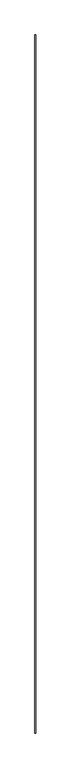
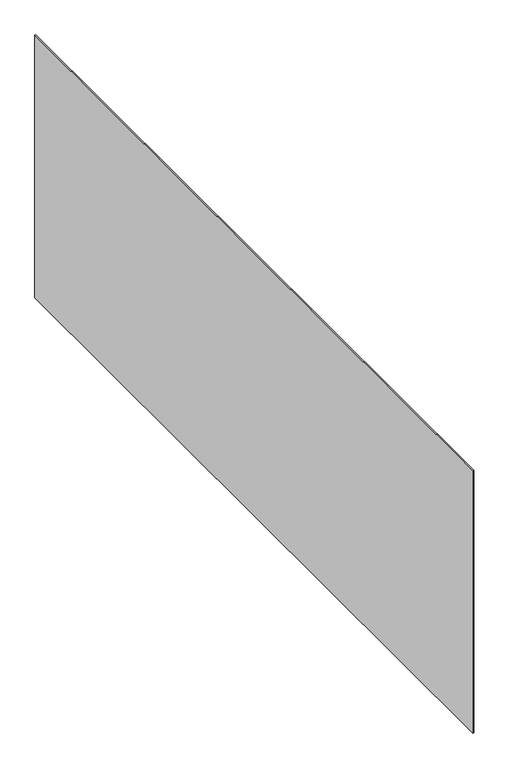
"""IFC4 building model written with IfcOpenShell, lengths in millimetres: proxy geometry, Panel:Panel:300402:Panel:300402 : Panel:Panel:300402:300124:Panel:300402:Panel:300402 : Panel:Panel:300402:300124 : Panel:Panel:300402:Panel:300402 : Panel:Panel:300402:300124:15 : Panel:Panel:300402:Panel:300402 : Panel:Panel:300402:300124:Panel:300402:Panel:300402 : Panel:Panel:300402:300124 : Panel:Panel:300402:Panel:300402 : Panel:Panel:300402:300124:300083."""

from ifc_helpers import new_model, si_unit, frame, origin, place, context, project, spatial, polyline, outline, extrude, source, transform, mapped, element, save


def generic_models_8c9edc3c(model_context):
    return source(origin(), model_context, "Body", "SweptSolid", [
        extrude(outline(polyline([(560264.0617239, -572944.1405465), (560264.0617239, -578718.1163841), (560256.1242239, -578718.1163841), (560256.1242239, -572944.1405465), (560264.0617239, -572944.1405465)])), frame((0.0, 0.0, 4023.758115), z_axis=(0.0, 0.0, 1.0), x_axis=(1.0, 0.0, 0.0)), (0.0, 0.0, 1.0), 2110.341885),
    ])


if __name__ == "__main__":
    model = new_model("IFC4")
    model_context = context("Model", 3, world=origin())
    ifc_project = project(units=[si_unit("LENGTHUNIT", "METRE", prefix="MILLI")], contexts=[model_context])
    site = spatial("IfcSite", under=ifc_project)
    building = spatial("IfcBuilding", under=site)
    placement = place(None, origin())
    generic_models_shape = generic_models_8c9edc3c(model_context)
    element("IfcBuildingElementProxy", 1, Name="Panel:Panel:300402:Panel:300402 : Panel:Panel:300402:300124:Panel:300402:Panel:300402 : Panel:Panel:300402:300124 : Panel:Panel:300402:Panel:300402 : Panel:Panel:300402:300124:15 : Panel:Panel:300402:Panel:300402 : Panel:Panel:300402:300124:Panel:300402:Panel:300402 : Panel:Panel:300402:300124 : Panel:Panel:300402:Panel:300402 : Panel:Panel:300402:300124:300083", ObjectType="Panel:Panel:300402:Panel:300402 : Panel:Panel:300402:300124:Panel:300402:Panel:300402 : Panel:Panel:300402:300124 : Panel:Panel:300402:Panel:300402 : Panel:Panel:300402:300124:15 : Panel:Panel:300402:Panel:300402 : Panel:Panel:300402:300124:Panel:300402:Panel:300402 : Panel:Panel:300402:300124 : Panel:Panel:300402:Panel:300402 : Panel:Panel:300402:300124:300083", at=placement, inside=building, context=model_context, shape_type="MappedRepresentation", body=[
        mapped(generic_models_shape, transform((0.0, 0.0, 0.0), x_axis=(1.0, 0.0, 0.0), y_axis=(0.0, 1.0, 0.0), z_axis=(0.0, 0.0, 1.0))),
    ])
    save(model, "model.ifc")

# Revit data of these elements
# Type "Panel:Panel:300402:Panel:300402 : Panel:Panel:300402:300124:Panel:300402:Panel:300402 : Panel:Panel:300402:300124 : Panel:Panel:300402:Panel:300402 : Panel:Panel:300402:300124:15 : Panel:Panel:300402:Panel:300402 : Panel:Panel:300402:300124:Panel:300402:Panel:300402 : Panel:Panel:300402:300124 : Panel:Panel:300402:Panel:300402 : Panel:Panel:300402:300124:300083"
#   NameOverride = "Panel:Panel:300402:Panel:300402 : Panel:Panel:300402:300124:Panel:300402:Panel:300402 : Panel:Panel:300402:300124 : Panel:Panel:300402:Panel:300402 : Panel:Panel:300402:300124:300083"
#   ObjectTypeOverride = "Panel:300402:Panel:300402 : Panel:Panel:300402:300124 : Panel:Panel:300402:Panel:300402 : Panel:Panel:300402:300124"
#   Reference = "Panel"
#   Tag = "300083"
# Element 1 (IfcBuildingElementProxy, "Panel:Panel:300402:Panel:300402 : Panel:Panel:300402:300124:Panel:300402:Panel:300402 : Panel:Panel:300402:300124 : Panel:Panel:300402:Panel:300402 : Panel:Panel:300402:300124:15 : Panel:Panel:300402:Panel:300402 : Panel:Panel:300402:300124:Panel:300402:Panel:300402 : Panel:Panel:300402:300124 : Panel:Panel:300402:Panel:300402 : Panel:Panel:300402:300124:300083")
#   Materials on its faces: "5/16\" THICK STONEWOOD RESIN PANELS - EXPOSED FASTENERS"
# Materials
#   "5/16\" THICK STONEWOOD RESIN PANELS - EXPOSED FASTENERS": class "Unassigned", colour RGB 64 64 64, transparency 0, Keynote = "M07420000.01", Cost = 0
